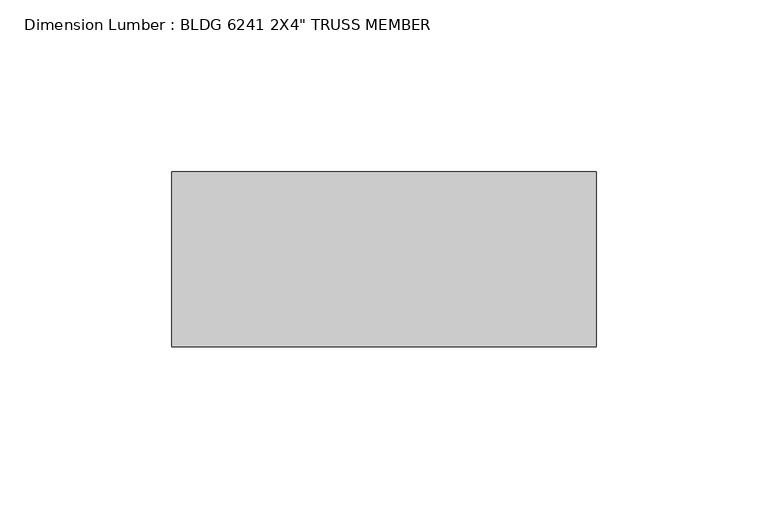
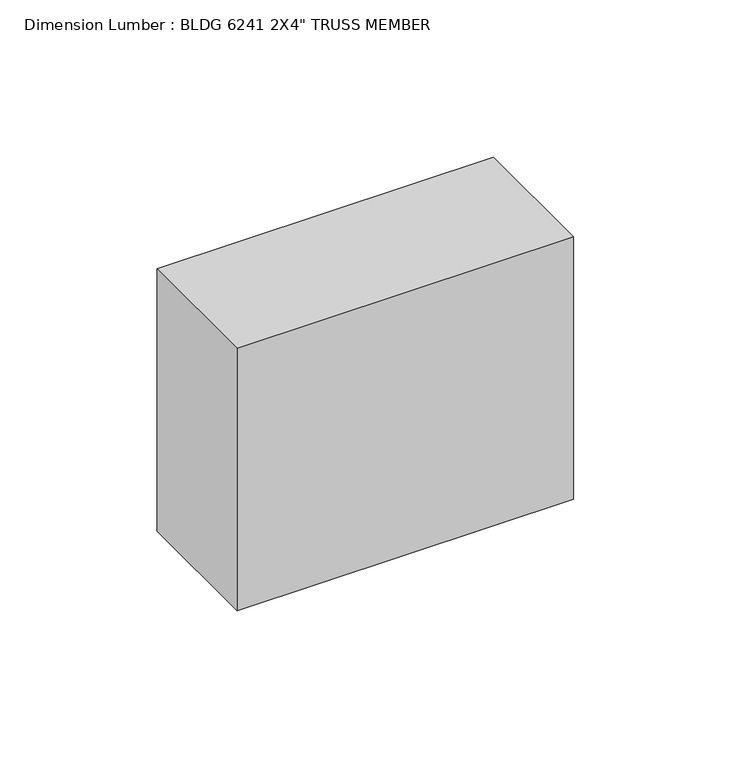
"""IFC4 building model written with IfcOpenShell, lengths in millimetres: beam geometry."""

from ifc_helpers import new_model, si_unit, frame, origin, place, context, project, spatial, polyline, outline, extrude, source, transform, mapped, element, save


def beam_878446a4(model_context):
    return source(origin(), model_context, "Body", "SweptSolid", [
        extrude(outline(polyline([(63.8057136, 25.4), (63.8057136, -25.4), (-59.553433, -25.4), (-59.553433, 25.4), (63.8057136, 25.4)])), frame((0.0, 0.0, -50.8), z_axis=(0.0, 0.0, 1.0), x_axis=(1.0, 0.0, 0.0)), (0.0, 0.0, 1.0), 101.6),
    ])


if __name__ == "__main__":
    model = new_model("IFC4")
    model_context = context("Model", 3, world=origin())
    ifc_project = project(units=[si_unit("LENGTHUNIT", "METRE", prefix="MILLI")], contexts=[model_context])
    site = spatial("IfcSite", under=ifc_project)
    building = spatial("IfcBuilding", under=site)
    placement = place(None, origin())
    beam_shape = beam_878446a4(model_context)
    element("IfcBeam", 1, ObjectType="Dimension Lumber : BLDG 6241 2X4\" TRUSS MEMBER", at=placement, inside=building, context=model_context, shape_type="MappedRepresentation", body=[
        mapped(beam_shape, transform((0.0, 0.0, 0.0), x_axis=(1.0, 0.0, 0.0), y_axis=(0.0, 1.0, 0.0), z_axis=(0.0, 0.0, 1.0))),
    ])
    save(model, "model.ifc")

# Revit data of these elements
# Type "Dimension Lumber : BLDG 6241 2X4\" TRUSS MEMBER"
#   Assembly Code = "B10"
#   A = 0.273472 SF
#   Length [instance default] = 5' - 0"
#   b = 0' - 2"
#   d = 0' - 4"
#   Structural Material [instance default] = Softwood, Lumber
# Element 1 (IfcBeam, "Dimension Lumber : BLDG 6241 2X4\" TRUSS MEMBER")
#   Materials on its faces: "Softwood, Lumber"
# Materials
#   "Softwood, Lumber": class "Wood", colour RGB 223 192 134, transparency 0, Description = "Pinus Echinata", Cost = 0
